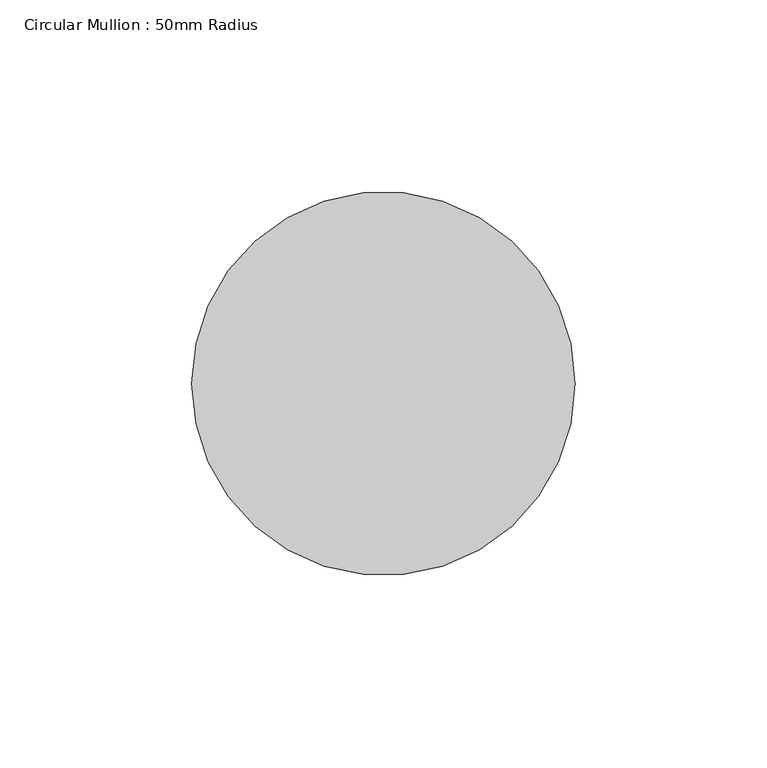
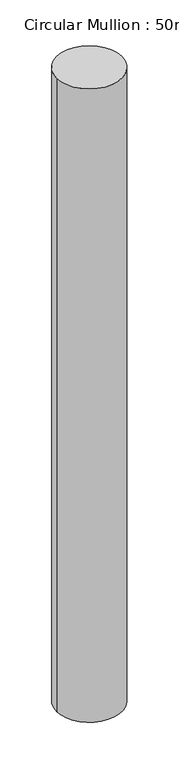
"""IFC4 building model written with IfcOpenShell, lengths in millimetres: member geometry, Circular Mullion : 50mm Radius."""

from ifc_helpers import new_model, si_unit, point, frame, origin, origin_2d, place, context, project, spatial, circle_curve, trimmed, segment, composite_curve, outline, extrude, source, transform, mapped, element, save


def circular_mullion_50mm_radius_955bb757(model_context):
    return source(origin(), model_context, "Body", "SweptSolid", [
        extrude(outline(composite_curve([segment(trimmed(circle_curve(origin_2d(), 50.0), [point((50.0, 0.0))], [point((-50.0, 0.0))], False, "CARTESIAN"), True, "CONTINUOUS"), segment(trimmed(circle_curve(origin_2d(), 50.0), [point((-50.0, 0.0))], [point((50.0, 0.0))], False, "CARTESIAN"), True, "CONTINUOUS")], self_intersect=False)), frame((0.0, 0.0, -1024.4312545), z_axis=(0.0, 0.0, 1.0), x_axis=(1.0, 0.0, 0.0)), (0.0, 0.0, 1.0), 1024.4312545),
    ])


if __name__ == "__main__":
    model = new_model("IFC4")
    model_context = context("Model", 3, world=origin())
    ifc_project = project(units=[si_unit("LENGTHUNIT", "METRE", prefix="MILLI")], contexts=[model_context])
    site = spatial("IfcSite", under=ifc_project)
    building = spatial("IfcBuilding", under=site)
    placement = place(None, origin())
    circular_mullion_50mm_radius_shape = circular_mullion_50mm_radius_955bb757(model_context)
    element("IfcMember", 1, ObjectType="Circular Mullion : 50mm Radius", at=placement, inside=building, context=model_context, shape_type="MappedRepresentation", body=[
        mapped(circular_mullion_50mm_radius_shape, transform((0.0, 0.0, 0.0), x_axis=(1.0, 0.0, 0.0), y_axis=(0.0, 1.0, 0.0), z_axis=(0.0, 0.0, 1.0))),
    ])
    save(model, "model.ifc")

# Revit data of these elements
# Type "Circular Mullion : 50mm Radius"
#   built-in parameter 1007350 = 0.164042 (stored number, unit not read)
# Element 1 (IfcMember, "Circular Mullion : 50mm Radius")
#   Materials on its faces: "Aluminium"
# Materials
#   "Aluminium": class "Metal", colour RGB 247 247 247, transparency 0, Description = "Aluminium 6061", Cost = 0
